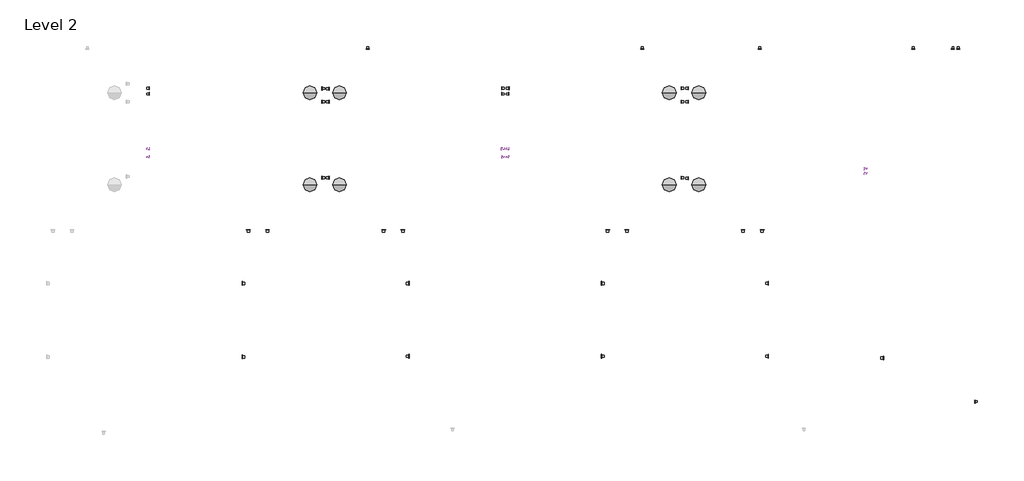
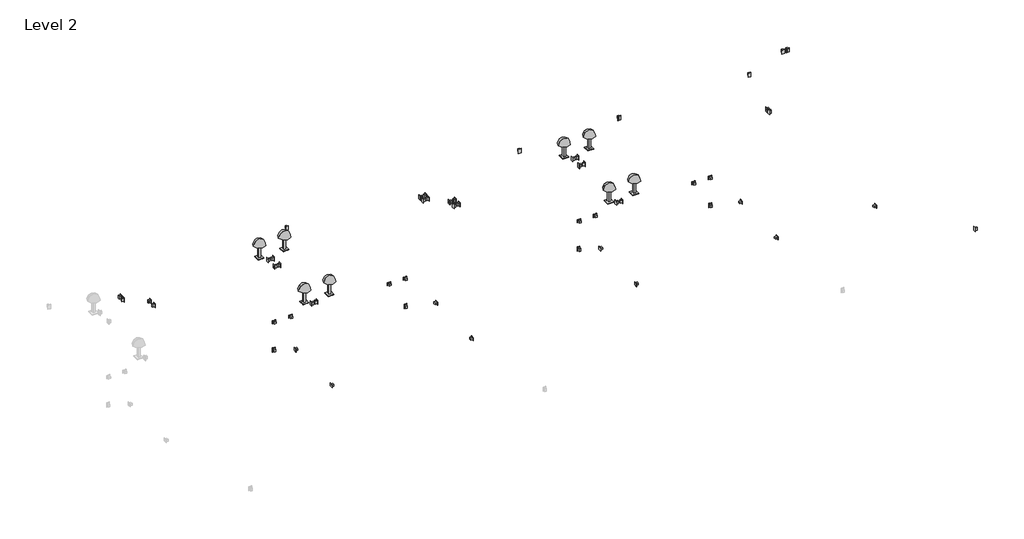
# One storey, part 2 of 2: 37 proxies, 17 switching devices, 8 light fixtures.
# Revit data of these elements (continued)
# Type "Table Lamp - Hemispheric : 60W - 230V" (continued)
#   built-in parameter 1150112 = 1 (stored number, unit not read)
#   built-in parameter 1150114 = 1 (stored number, unit not read)
#   built-in parameter 1150107 = 2800 (stored number, unit not read)
#   built-in parameter 1150106 = 0.680387 (stored number, unit not read)
#   built-in parameter 1150104 = 1.32387 (stored number, unit not read)
#   Ballast Voltage = 230 V
#   built-in parameter 1114218 = 1 (stored number, unit not read)
#   built-in parameter 1150133 = 10 (stored number, unit not read)
#   Lumens = 855 lm
#   Apparent Load = 60 VA
#   COBie.Type = yes
#   built-in parameter 1150134 = 4
#   built-in parameter 1150137 = 1
#   Color Filter = 16777215
#   Ballast Number of Poles = 1
#   T.L. Material = Wood - Birch
#   Mount Material = Metal - Chrome
#   Load Classification = Lighting - Dwelling Unit
#   Shade Material = Glass - Frosted
#   Base Material = Wood - Birch
#   Dimming Lamp Color Temperature Shift = (empty or 0)
#   Default Elevation = 0
#   Wattage Comments = ""
# Type "Lighting Switches One Way : One Way Switch"
#   Type Mark = "Lighting Switches One Way"
#   Classification.OmniClass.21.Number = "21-04 50 40 10"
#   Classification.OmniClass.21.Description = "Lighting Control"
#   Classification.UniFormat.II.Description = "Lighting Control"
#   Classification.OmniClass.23.Number = "23-35 37 00"
#   Classification.OmniClass.23.Description = "Electrical Switches"
#   Classification.UniFormat.II.Number = "D5040.10"
#   COBie.Type.CreatedBy = "info@mma.ie"
#   COBie.Type.CreatedOn = "2017-07-25T10:15:16"
#   COBie.Type.Name = "Lighting Switches One Way"
#   COBie.Type.Category = "23-35 37 00 : Electrical Switches"
#   COBie.Type.Description = "Lighting Switches One Way_One Way Switch"
#   COBie.Type.AssetType = "Fixed"
#   COBie.Type.Manufacturer = ""
#   COBie.Type.ModelNumber = ""
#   Label = ""
#   Keynote = "26 36 13.A"
#   COBie.Type.ReplacementCost = 0
#   Switch Voltage [instance default] = 230 V
#   Default Elevation = 1200 mm
#   Apparent Load = 0 VA
#   1.W.S. Width = 86 mm
#   1.W.S. Height = 86 mm
#   1.W.S. Depth = 59 mm
#   COBie.Type = yes
#   Visibility 7 = no
#   Visibility 6 = no
#   Visibility 5 = yes
#   Visibility 4 = no
#   Visibility 3 = no
#   Visibility 2 = no
#   Visibility 1 = no
#   Ballast Number of Poles = 1
#   Load Classification = Other
#   1.W.S. Material = Metal - Chrome
# Type "Lighting Switches Two Way : Two Way Switch"
#   Type Mark = "Lighting Switches Two Way"
#   Classification.OmniClass.23.Number = "23-35 37 00"
#   Classification.OmniClass.23.Description = "Electrical Switches"
#   COBie.Type.CreatedBy = "info@mma.ie"
#   COBie.Type.CreatedOn = "2017-07-25T10:15:16"
#   COBie.Type.Name = "Lighting Switches Two Way"
#   COBie.Type.Category = "23-35 37 00 : Electrical Switches"
#   COBie.Type.Description = "Lighting Switches Two Way_Two Way Switch"
#   COBie.Type.AssetType = "Fixed"
#   COBie.Type.Manufacturer = ""
#   COBie.Type.ModelNumber = ""
#   Label = ""
#   Keynote = "26 36 13.B"
#   COBie.Type.ReplacementCost = 0
#   Switch Voltage [instance default] = 230 V
#   Default Elevation = 1200 mm
#   Apparent Load = 0 VA
#   2.W.S. Width = 86 mm
#   2.W.S. Height = 86 mm
#   2.W.S. Depth = 59 mm
#   COBie.Type = yes
#   Visibility 7 = no
#   Visibility 6 = no
#   Visibility 5 = yes
#   Visibility 4 = no
#   Visibility 3 = no
#   Visibility 2 = no
#   Visibility 1 = no
#   Ballast Number of Poles = 1
#   Load Classification = Other
#   2.W.S. Material = Metal - Chrome
# Element 1 (IfcBuildingElementProxy, "M_Duplex Receptacle - Top Switched : Standard")
#   Mark = "1"
#   COBie.CreatedBy = "info@mma.ie"
#   COBie.CreatedOn = "2017-07-25T10:15:16"
#   COBie.Component.Name = "M_Duplex Receptacle - Top Switched_1"
#   COBie.Component.Space = "213"
#   COBie.Component.Description = "M_Duplex Receptacle - Top Switched: Standard"
#   Notes = "n/a"
#   COBie = yes
#   Phase Created = New Construction
# Element 2 (IfcBuildingElementProxy, "M_Duplex Receptacle - Top Switched : Standard")
#   Mark = "2"
#   COBie.CreatedBy = "info@mma.ie"
#   COBie.CreatedOn = "2017-07-25T10:15:16"
#   COBie.Component.Name = "M_Duplex Receptacle - Top Switched_2"
#   COBie.Component.Space = "215"
#   COBie.Component.Description = "M_Duplex Receptacle - Top Switched: Standard"
#   Notes = "n/a"
#   COBie = yes
#   Phase Created = New Construction
# Element 3 (IfcBuildingElementProxy, "M_Duplex Receptacle - Top Switched : Standard")
#   Mark = "3"
#   COBie.CreatedBy = "info@mma.ie"
#   COBie.CreatedOn = "2017-07-25T10:15:16"
#   COBie.Component.Name = "M_Duplex Receptacle - Top Switched_3"
#   COBie.Component.Space = "215"
#   COBie.Component.Description = "M_Duplex Receptacle - Top Switched: Standard"
#   Notes = "n/a"
#   COBie = yes
#   Phase Created = New Construction
# Element 4 (IfcBuildingElementProxy, "M_Duplex Receptacle - Top Switched : Standard")
#   Mark = "4"
#   COBie.CreatedBy = "info@mma.ie"
#   COBie.CreatedOn = "2017-07-25T10:15:16"
#   COBie.Component.Name = "M_Duplex Receptacle - Top Switched_4"
#   COBie.Component.Space = "211"
#   COBie.Component.Description = "M_Duplex Receptacle - Top Switched: Standard"
#   Notes = "n/a"
#   COBie = yes
#   Phase Created = New Construction
# Element 5 (IfcBuildingElementProxy, "M_Duplex Receptacle - Top Switched : Standard")
#   Mark = "5"
#   COBie.CreatedBy = "info@mma.ie"
#   COBie.CreatedOn = "2017-07-25T10:15:16"
#   COBie.Component.Name = "M_Duplex Receptacle - Top Switched_5"
#   COBie.Component.Space = "211"
#   COBie.Component.Description = "M_Duplex Receptacle - Top Switched: Standard"
#   Notes = "n/a"
#   COBie = yes
#   Phase Created = New Construction
# Element 6 (IfcBuildingElementProxy, "M_Duplex Receptacle - Top Switched : Standard")
#   Mark = "6"
#   COBie.CreatedBy = "info@mma.ie"
#   COBie.CreatedOn = "2017-07-25T10:15:16"
#   COBie.Component.Name = "M_Duplex Receptacle - Top Switched_6"
#   COBie.Component.Space = "209"
#   COBie.Component.Description = "M_Duplex Receptacle - Top Switched: Standard"
#   Notes = "n/a"
#   COBie = yes
#   Phase Created = New Construction
# Element 7 (IfcBuildingElementProxy, "M_Duplex Receptacle - Top Switched : Standard")
#   Mark = "11"
#   COBie.CreatedBy = "info@mma.ie"
#   COBie.CreatedOn = "2017-07-25T10:15:16"
#   COBie.Component.Name = "M_Duplex Receptacle - Top Switched_11"
#   COBie.Component.Space = "209"
#   COBie.Component.Description = "M_Duplex Receptacle - Top Switched: Standard"
#   Notes = "n/a"
#   COBie = yes
#   Phase Created = New Construction
# Element 8 (IfcBuildingElementProxy, "M_Duplex Receptacle - Top Switched : Standard")
#   Mark = "12"
#   COBie.CreatedBy = "info@mma.ie"
#   COBie.CreatedOn = "2017-07-25T10:15:16"
#   COBie.Component.Name = "M_Duplex Receptacle - Top Switched_12"
#   COBie.Component.Space = "213"
#   COBie.Component.Description = "M_Duplex Receptacle - Top Switched: Standard"
#   Notes = "n/a"
#   COBie = yes
#   Phase Created = New Construction
# Element 9 (IfcBuildingElementProxy, "M_Duplex Receptacle - Top Switched : Standard")
#   Mark = "13"
#   COBie.CreatedBy = "info@mma.ie"
#   COBie.CreatedOn = "2017-07-25T10:15:16"
#   COBie.Component.Name = "M_Duplex Receptacle - Top Switched_13"
#   COBie.Component.Space = "213"
#   COBie.Component.Description = "M_Duplex Receptacle - Top Switched: Standard"
#   Notes = "n/a"
#   COBie = yes
#   Phase Created = New Construction
# Element 10 (IfcBuildingElementProxy, "M_Duplex Receptacle - Top Switched : Standard")
#   Mark = "14"
#   COBie.CreatedBy = "info@mma.ie"
#   COBie.CreatedOn = "2017-07-25T10:15:16"
#   COBie.Component.Name = "M_Duplex Receptacle - Top Switched_14"
#   COBie.Component.Space = "215"
#   COBie.Component.Description = "M_Duplex Receptacle - Top Switched: Standard"
#   Notes = "n/a"
#   COBie = yes
#   Phase Created = New Construction
# Element 11 (IfcBuildingElementProxy, "M_Receptacle - 220V : Standard")
#   Mark = "1"
#   COBie.CreatedBy = "info@mma.ie"
#   COBie.CreatedOn = "2017-07-25T10:15:16"
#   COBie.Component.Name = "M_Receptacle - 220V_1"
#   COBie.Component.Space = "215"
#   COBie.Component.Description = "M_Receptacle - 220V: Standard"
#   Notes = "n/a"
#   COBie = yes
#   Phase Created = New Construction
# Element 12 (IfcBuildingElementProxy, "M_Receptacle - 220V : Standard")
#   Mark = "2"
#   COBie.CreatedBy = "info@mma.ie"
#   COBie.CreatedOn = "2017-07-25T10:15:16"
#   COBie.Component.Name = "M_Receptacle - 220V_2"
#   COBie.Component.Space = "215"
#   COBie.Component.Description = "M_Receptacle - 220V: Standard"
#   Notes = "n/a"
#   COBie = yes
#   Phase Created = New Construction
# Element 13 (IfcBuildingElementProxy, "M_Receptacle - 220V : Standard")
#   Mark = "3"
#   COBie.CreatedBy = "info@mma.ie"
#   COBie.CreatedOn = "2017-07-25T10:15:16"
#   COBie.Component.Name = "M_Receptacle - 220V_3"
#   COBie.Component.Space = "215"
#   COBie.Component.Description = "M_Receptacle - 220V: Standard"
#   Notes = "n/a"
#   COBie = yes
#   Phase Created = New Construction
# Element 14 (IfcBuildingElementProxy, "M_Receptacle - 220V : Standard")
#   Mark = "4"
#   COBie.CreatedBy = "info@mma.ie"
#   COBie.CreatedOn = "2017-07-25T10:15:16"
#   COBie.Component.Name = "M_Receptacle - 220V_4"
#   COBie.Component.Space = "215"
#   COBie.Component.Description = "M_Receptacle - 220V: Standard"
#   Notes = "n/a"
#   COBie = yes
#   Phase Created = New Construction
# Element 15 (IfcBuildingElementProxy, "M_Receptacle - 220V : Standard")
#   Mark = "5"
#   COBie.CreatedBy = "info@mma.ie"
#   COBie.CreatedOn = "2017-07-25T10:15:16"
#   COBie.Component.Name = "M_Receptacle - 220V_5"
#   COBie.Component.Space = "213"
#   COBie.Component.Description = "M_Receptacle - 220V: Standard"
#   Notes = "n/a"
#   COBie = yes
#   Phase Created = New Construction
# Element 16 (IfcBuildingElementProxy, "M_Receptacle - 220V : Standard")
#   Mark = "6"
#   COBie.CreatedBy = "info@mma.ie"
#   COBie.CreatedOn = "2017-07-25T10:15:16"
#   COBie.Component.Name = "M_Receptacle - 220V_6"
#   COBie.Component.Space = "213"
#   COBie.Component.Description = "M_Receptacle - 220V: Standard"
#   Notes = "n/a"
#   COBie = yes
#   Phase Created = New Construction
# Element 17 (IfcBuildingElementProxy, "M_Receptacle - 220V : Standard")
#   Mark = "7"
#   COBie.CreatedBy = "info@mma.ie"
#   COBie.CreatedOn = "2017-07-25T10:15:16"
#   COBie.Component.Name = "M_Receptacle - 220V_7"
#   COBie.Component.Space = "213"
#   COBie.Component.Description = "M_Receptacle - 220V: Standard"
#   Notes = "n/a"
#   COBie = yes
#   Phase Created = New Construction
# Element 18 (IfcBuildingElementProxy, "M_Receptacle - 220V : Standard")
#   Mark = "8"
#   COBie.CreatedBy = "info@mma.ie"
#   COBie.CreatedOn = "2017-07-25T10:15:16"
#   COBie.Component.Name = "M_Receptacle - 220V_8"
#   COBie.Component.Space = "211"
#   COBie.Component.Description = "M_Receptacle - 220V: Standard"
#   Notes = "n/a"
#   COBie = yes
#   Phase Created = New Construction
# Element 19 (IfcBuildingElementProxy, "M_Receptacle - 220V : Standard")
#   Mark = "9"
#   COBie.CreatedBy = "info@mma.ie"
#   COBie.CreatedOn = "2017-07-25T10:15:16"
#   COBie.Component.Name = "M_Receptacle - 220V_9"
#   COBie.Component.Space = "211"
#   COBie.Component.Description = "M_Receptacle - 220V: Standard"
#   Notes = "n/a"
#   COBie = yes
#   Phase Created = New Construction
# Element 20 (IfcBuildingElementProxy, "M_Receptacle - 220V : Standard")
#   Mark = "10"
#   COBie.CreatedBy = "info@mma.ie"
#   COBie.CreatedOn = "2017-07-25T10:15:16"
#   COBie.Component.Name = "M_Receptacle - 220V_10"
#   COBie.Component.Space = "211"
#   COBie.Component.Description = "M_Receptacle - 220V: Standard"
#   Notes = "n/a"
#   COBie = yes
#   Phase Created = New Construction
# Element 21 (IfcBuildingElementProxy, "M_Receptacle - 220V : Standard")
#   Mark = "11"
#   COBie.CreatedBy = "info@mma.ie"
#   COBie.CreatedOn = "2017-07-25T10:15:16"
#   COBie.Component.Name = "M_Receptacle - 220V_11"
#   COBie.Component.Space = "211"
#   COBie.Component.Description = "M_Receptacle - 220V: Standard"
#   Notes = "n/a"
#   COBie = yes
#   Phase Created = New Construction
# Element 22 (IfcBuildingElementProxy, "M_Receptacle - 220V : Standard")
#   Mark = "12"
#   COBie.CreatedBy = "info@mma.ie"
#   COBie.CreatedOn = "2017-07-25T10:15:16"
#   COBie.Component.Name = "M_Receptacle - 220V_12"
#   COBie.Component.Space = "209"
#   COBie.Component.Description = "M_Receptacle - 220V: Standard"
#   Notes = "n/a"
#   COBie = yes
#   Phase Created = New Construction
# Element 23 (IfcBuildingElementProxy, "M_Receptacle - 220V : Standard")
#   Mark = "13"
#   COBie.CreatedBy = "info@mma.ie"
#   COBie.CreatedOn = "2017-07-25T10:15:16"
#   COBie.Component.Name = "M_Receptacle - 220V_13"
#   COBie.Component.Space = "209"
#   COBie.Component.Description = "M_Receptacle - 220V: Standard"
#   Notes = "n/a"
#   COBie = yes
#   Phase Created = New Construction
# Element 24 (IfcBuildingElementProxy, "M_Receptacle - 220V : Standard")
#   Mark = "14"
#   COBie.CreatedBy = "info@mma.ie"
#   COBie.CreatedOn = "2017-07-25T10:15:16"
#   COBie.Component.Name = "M_Receptacle - 220V_14"
#   COBie.Component.Space = "209"
#   COBie.Component.Description = "M_Receptacle - 220V: Standard"
#   Notes = "n/a"
#   COBie = yes
#   Phase Created = New Construction
# Element 25 (IfcBuildingElementProxy, "M_Receptacle - 220V : Standard")
#   Mark = "37"
#   COBie.CreatedBy = "info@mma.ie"
#   COBie.CreatedOn = "2017-07-25T10:15:16"
#   COBie.Component.Name = "M_Receptacle - 220V_37"
#   COBie.Component.Space = "219"
#   COBie.Component.Description = "M_Receptacle - 220V: Standard"
#   Notes = "n/a"
#   COBie = yes
#   Phase Created = New Construction
# Element 26 (IfcBuildingElementProxy, "M_Receptacle - DATA socket : Standard")
#   Mark = "6"
#   COBie.CreatedBy = "info@mma.ie"
#   COBie.CreatedOn = "2017-07-25T10:15:16"
#   COBie.Component.Name = "M_Receptacle - DATA socket_6"
#   COBie.Component.Space = "209"
#   COBie.Component.Description = "M_Receptacle - DATA socket: Standard"
#   Notes = "n/a"
#   COBie = yes
#   Phase Created = New Construction
# Element 27 (IfcBuildingElementProxy, "M_Receptacle - DATA socket : Standard")
#   Mark = "7"
#   COBie.CreatedBy = "info@mma.ie"
#   COBie.CreatedOn = "2017-07-25T10:15:16"
#   COBie.Component.Name = "M_Receptacle - DATA socket_7"
#   COBie.Component.Space = "209"
#   COBie.Component.Description = "M_Receptacle - DATA socket: Standard"
#   Notes = "n/a"
#   COBie = yes
#   Phase Created = New Construction
# Element 28 (IfcBuildingElementProxy, "M_Receptacle - DATA socket : Standard")
#   Mark = "8"
#   COBie.CreatedBy = "info@mma.ie"
#   COBie.CreatedOn = "2017-07-25T10:15:16"
#   COBie.Component.Name = "M_Receptacle - DATA socket_8"
#   COBie.Component.Space = "211"
#   COBie.Component.Description = "M_Receptacle - DATA socket: Standard"
#   Notes = "n/a"
#   COBie = yes
#   Phase Created = New Construction
# Element 29 (IfcBuildingElementProxy, "M_Receptacle - DATA socket : Standard")
#   Mark = "9"
#   COBie.CreatedBy = "info@mma.ie"
#   COBie.CreatedOn = "2017-07-25T10:15:16"
#   COBie.Component.Name = "M_Receptacle - DATA socket_9"
#   COBie.Component.Space = "211"
#   COBie.Component.Description = "M_Receptacle - DATA socket: Standard"
#   Notes = "n/a"
#   COBie = yes
#   Phase Created = New Construction
# Element 30 (IfcBuildingElementProxy, "M_Receptacle - DATA socket : Standard")
#   Mark = "10"
#   COBie.CreatedBy = "info@mma.ie"
#   COBie.CreatedOn = "2017-07-25T10:15:16"
#   COBie.Component.Name = "M_Receptacle - DATA socket_10"
#   COBie.Component.Space = "213"
#   COBie.Component.Description = "M_Receptacle - DATA socket: Standard"
#   Notes = "n/a"
#   COBie = yes
#   Phase Created = New Construction
# Element 31 (IfcBuildingElementProxy, "M_Receptacle - DATA socket : Standard")
#   Mark = "11"
#   COBie.CreatedBy = "info@mma.ie"
#   COBie.CreatedOn = "2017-07-25T10:15:16"
#   COBie.Component.Name = "M_Receptacle - DATA socket_11"
#   COBie.Component.Space = "215"
#   COBie.Component.Description = "M_Receptacle - DATA socket: Standard"
#   Notes = "n/a"
#   COBie = yes
#   Phase Created = New Construction
# Element 32 (IfcBuildingElementProxy, "M_Receptacle - DATA socket : Standard")
#   Mark = "18"
#   COBie.CreatedBy = "info@mma.ie"
#   COBie.CreatedOn = "2017-07-25T10:15:16"
#   COBie.Component.Name = "M_Receptacle - DATA socket_18"
#   COBie.Component.Space = "213"
#   COBie.Component.Description = "M_Receptacle - DATA socket: Standard"
#   Notes = "n/a"
#   COBie = yes
#   Phase Created = New Construction
# Element 33 (IfcBuildingElementProxy, "M_Receptacle - DATA socket : Standard")
#   Mark = "21"
#   COBie.CreatedBy = "info@mma.ie"
#   COBie.CreatedOn = "2017-07-25T10:15:16"
#   COBie.Component.Name = "M_Receptacle - DATA socket_21"
#   COBie.Component.Space = "215"
#   COBie.Component.Description = "M_Receptacle - DATA socket: Standard"
#   Notes = "n/a"
#   COBie = yes
#   Phase Created = New Construction
# Element 34 (IfcBuildingElementProxy, "M_Receptacle -TV /Satellite Socket : Standard")
#   Mark = "3"
#   COBie.CreatedBy = "info@mma.ie"
#   COBie.CreatedOn = "2017-07-25T10:15:16"
#   COBie.Component.Name = "M_Receptacle -TV_3"
#   COBie.Component.Space = "211"
#   COBie.Component.Description = "M_Receptacle -TV: Standard"
#   Notes = "n/a"
#   COBie = yes
#   Phase Created = New Construction
# Element 35 (IfcBuildingElementProxy, "M_Receptacle -TV /Satellite Socket : Standard")
#   Mark = "4"
#   COBie.CreatedBy = "info@mma.ie"
#   COBie.CreatedOn = "2017-07-25T10:15:16"
#   COBie.Component.Name = "M_Receptacle -TV_4"
#   COBie.Component.Space = "213"
#   COBie.Component.Description = "M_Receptacle -TV: Standard"
#   Notes = "n/a"
#   COBie = yes
#   Phase Created = New Construction
# Element 36 (IfcBuildingElementProxy, "M_Receptacle -TV /Satellite Socket : Standard")
#   Mark = "5"
#   COBie.CreatedBy = "info@mma.ie"
#   COBie.CreatedOn = "2017-07-25T10:15:16"
#   COBie.Component.Name = "M_Receptacle -TV_5"
#   COBie.Component.Space = "215"
#   COBie.Component.Description = "M_Receptacle -TV: Standard"
#   Notes = "n/a"
#   COBie = yes
#   Phase Created = New Construction
# Element 37 (IfcBuildingElementProxy, "M_Receptacle -TV /Satellite Socket : Standard")
#   Mark = "6"
#   COBie.CreatedBy = "info@mma.ie"
#   COBie.CreatedOn = "2017-07-25T10:15:16"
#   COBie.Component.Name = "M_Receptacle -TV_6"
#   COBie.Component.Space = "209"
#   COBie.Component.Description = "M_Receptacle -TV: Standard"
#   Notes = "n/a"
#   COBie = yes
#   Phase Created = New Construction
# Element 38 (IfcLightFixture, "Table Lamp - Hemispheric : 60W - 230V")
#   Comments = "Lamps"
#   Mark = "1"
#   COBie.CreatedBy = "info@mma.ie"
#   COBie.CreatedOn = "2017-07-25T10:15:16"
#   COBie.Component.Name = "Table Lamp - Hemispheric_1"
#   COBie.Component.Space = "211"
#   COBie.Component.Description = "Table Lamp - Hemispheric: 60W - 230V"
#   Notes = "n/a"
#   Floor Level = "Level 2"
#   COBie = yes
#   Phase Created = New Construction
#   Materials on its faces: "Metal - Chrome", "Glass - Frosted", "Wood - Birch"
# Element 39 (IfcLightFixture, "Table Lamp - Hemispheric : 60W - 230V")
#   Comments = "Lamps"
#   Mark = "2"
#   COBie.CreatedBy = "info@mma.ie"
#   COBie.CreatedOn = "2017-07-25T10:15:16"
#   COBie.Component.Name = "Table Lamp - Hemispheric_2"
#   COBie.Component.Space = "211"
#   COBie.Component.Description = "Table Lamp - Hemispheric: 60W - 230V"
#   Notes = "n/a"
#   Floor Level = "Level 2"
#   COBie = yes
#   Phase Created = New Construction
#   Materials on its faces: "Metal - Chrome", "Glass - Frosted", "Wood - Birch"
# Element 40 (IfcLightFixture, "Table Lamp - Hemispheric : 60W - 230V")
#   Comments = "Lamps"
#   Mark = "3"
#   COBie.CreatedBy = "info@mma.ie"
#   COBie.CreatedOn = "2017-07-25T10:15:16"
#   COBie.Component.Name = "Table Lamp - Hemispheric_3"
#   COBie.Component.Space = "209"
#   COBie.Component.Description = "Table Lamp - Hemispheric: 60W - 230V"
#   Notes = "n/a"
#   Floor Level = "Level 2"
#   COBie = yes
#   Phase Created = New Construction
#   Materials on its faces: "Metal - Chrome", "Glass - Frosted", "Wood - Birch"
# Element 41 (IfcLightFixture, "Table Lamp - Hemispheric : 60W - 230V")
#   Comments = "Lamps"
#   Mark = "4"
#   COBie.CreatedBy = "info@mma.ie"
#   COBie.CreatedOn = "2017-07-25T10:15:16"
#   COBie.Component.Name = "Table Lamp - Hemispheric_4"
#   COBie.Component.Space = "209"
#   COBie.Component.Description = "Table Lamp - Hemispheric: 60W - 230V"
#   Notes = "n/a"
#   Floor Level = "Level 2"
#   COBie = yes
#   Phase Created = New Construction
#   Materials on its faces: "Metal - Chrome", "Glass - Frosted", "Wood - Birch"
# Element 42 (IfcLightFixture, "Table Lamp - Hemispheric : 60W - 230V")
#   Comments = "Lamps"
#   Mark = "11"
#   COBie.CreatedBy = "info@mma.ie"
#   COBie.CreatedOn = "2017-07-25T10:15:16"
#   COBie.Component.Name = "Table Lamp - Hemispheric_11"
#   COBie.Component.Space = "213"
#   COBie.Component.Description = "Table Lamp - Hemispheric: 60W - 230V"
#   Notes = "n/a"
#   Floor Level = "Level 2"
#   COBie = yes
#   Phase Created = New Construction
#   Materials on its faces: "Metal - Chrome", "Glass - Frosted", "Wood - Birch"
# Element 43 (IfcLightFixture, "Table Lamp - Hemispheric : 60W - 230V")
#   Comments = "Lamps"
#   Mark = "12"
#   COBie.CreatedBy = "info@mma.ie"
#   COBie.CreatedOn = "2017-07-25T10:15:16"
#   COBie.Component.Name = "Table Lamp - Hemispheric_12"
#   COBie.Component.Space = "213"
#   COBie.Component.Description = "Table Lamp - Hemispheric: 60W - 230V"
#   Notes = "n/a"
#   Floor Level = "Level 2"
#   COBie = yes
#   Phase Created = New Construction
#   Materials on its faces: "Metal - Chrome", "Glass - Frosted", "Wood - Birch"
# Element 44 (IfcLightFixture, "Table Lamp - Hemispheric : 60W - 230V")
#   Comments = "Lamps"
#   Mark = "13"
#   COBie.CreatedBy = "info@mma.ie"
#   COBie.CreatedOn = "2017-07-25T10:15:16"
#   COBie.Component.Name = "Table Lamp - Hemispheric_13"
#   COBie.Component.Space = "215"
#   COBie.Component.Description = "Table Lamp - Hemispheric: 60W - 230V"
#   Notes = "n/a"
#   Floor Level = "Level 2"
#   COBie = yes
#   Phase Created = New Construction
#   Materials on its faces: "Metal - Chrome", "Glass - Frosted", "Wood - Birch"
# Element 45 (IfcLightFixture, "Table Lamp - Hemispheric : 60W - 230V")
#   Comments = "Lamps"
#   Mark = "14"
#   COBie.CreatedBy = "info@mma.ie"
#   COBie.CreatedOn = "2017-07-25T10:15:16"
#   COBie.Component.Name = "Table Lamp - Hemispheric_14"
#   COBie.Component.Space = "215"
#   COBie.Component.Description = "Table Lamp - Hemispheric: 60W - 230V"
#   Notes = "n/a"
#   Floor Level = "Level 2"
#   COBie = yes
#   Phase Created = New Construction
#   Materials on its faces: "Metal - Chrome", "Glass - Frosted", "Wood - Birch"
# Element 46 (IfcSwitchingDevice, "Lighting Switches One Way : One Way Switch")
#   Comments = "Switch"
#   Mark = "10"
#   COBie.CreatedBy = "info@mma.ie"
#   COBie.CreatedOn = "2017-07-25T10:15:16"
#   COBie.Component.Name = "Lighting Switches One Way_10"
#   COBie.Component.Space = "213"
#   COBie.Component.Description = "Lighting Switches One Way: One Way Switch"
#   Notes = "n/a"
#   Floor Level = "Level 2"
#   COBie = yes
#   Phase Created = New Construction
# Element 47 (IfcSwitchingDevice, "Lighting Switches One Way : One Way Switch")
#   Comments = "Switch"
#   Mark = "11"
#   COBie.CreatedBy = "info@mma.ie"
#   COBie.CreatedOn = "2017-07-25T10:15:16"
#   COBie.Component.Name = "Lighting Switches One Way_11"
#   COBie.Component.Space = "215"
#   COBie.Component.Description = "Lighting Switches One Way: One Way Switch"
#   Notes = "n/a"
#   Floor Level = "Level 2"
#   COBie = yes
#   Phase Created = New Construction
# Element 48 (IfcSwitchingDevice, "Lighting Switches One Way : One Way Switch")
#   Comments = "Switch"
#   Mark = "12"
#   COBie.CreatedBy = "info@mma.ie"
#   COBie.CreatedOn = "2017-07-25T10:15:16"
#   COBie.Component.Name = "Lighting Switches One Way_12"
#   COBie.Component.Space = "211"
#   COBie.Component.Description = "Lighting Switches One Way: One Way Switch"
#   Notes = "n/a"
#   Floor Level = "Level 2"
#   COBie = yes
#   Phase Created = New Construction
# Element 49 (IfcSwitchingDevice, "Lighting Switches One Way : One Way Switch")
#   Comments = "Switch"
#   Mark = "13"
#   COBie.CreatedBy = "info@mma.ie"
#   COBie.CreatedOn = "2017-07-25T10:15:16"
#   COBie.Component.Name = "Lighting Switches One Way_13"
#   COBie.Component.Space = "209"
#   COBie.Component.Description = "Lighting Switches One Way: One Way Switch"
#   Notes = "n/a"
#   Floor Level = "Level 2"
#   COBie = yes
#   Phase Created = New Construction
# Element 50 (IfcSwitchingDevice, "Lighting Switches One Way : One Way Switch")
#   Comments = "Switch"
#   Mark = "16"
#   COBie.CreatedBy = "info@mma.ie"
#   COBie.CreatedOn = "2017-07-25T10:15:16"
#   COBie.Component.Name = "Lighting Switches One Way_16"
#   COBie.Component.Space = "209"
#   COBie.Component.Description = "Lighting Switches One Way: One Way Switch"
#   Notes = "n/a"
#   Floor Level = "Level 2"
#   COBie = yes
#   Phase Created = New Construction
# Element 51 (IfcSwitchingDevice, "Lighting Switches One Way : One Way Switch")
#   Comments = "Switch"
#   Mark = "17"
#   COBie.CreatedBy = "info@mma.ie"
#   COBie.CreatedOn = "2017-07-25T10:15:16"
#   COBie.Component.Name = "Lighting Switches One Way_17"
#   COBie.Component.Space = "209"
#   COBie.Component.Description = "Lighting Switches One Way: One Way Switch"
#   Notes = "n/a"
#   Floor Level = "Level 2"
#   COBie = yes
#   Phase Created = New Construction
# Element 52 (IfcSwitchingDevice, "Lighting Switches One Way : One Way Switch")
#   Comments = "Switch"
#   Mark = "18"
#   COBie.CreatedBy = "info@mma.ie"
#   COBie.CreatedOn = "2017-07-25T10:15:16"
#   COBie.Component.Name = "Lighting Switches One Way_18"
#   COBie.Component.Space = "213"
#   COBie.Component.Description = "Lighting Switches One Way: One Way Switch"
#   Notes = "n/a"
#   Floor Level = "Level 2"
#   COBie = yes
#   Phase Created = New Construction
# Element 53 (IfcSwitchingDevice, "Lighting Switches One Way : One Way Switch")
#   Comments = "Switch"
#   Mark = "19"
#   COBie.CreatedBy = "info@mma.ie"
#   COBie.CreatedOn = "2017-07-25T10:15:16"
#   COBie.Component.Name = "Lighting Switches One Way_19"
#   COBie.Component.Space = "215"
#   COBie.Component.Description = "Lighting Switches One Way: One Way Switch"
#   Notes = "n/a"
#   Floor Level = "Level 2"
#   COBie = yes
#   Phase Created = New Construction
# Element 54 (IfcSwitchingDevice, "Lighting Switches One Way : One Way Switch")
#   Comments = "Switch"
#   Mark = "20"
#   COBie.CreatedBy = "info@mma.ie"
#   COBie.CreatedOn = "2017-07-25T10:15:16"
#   COBie.Component.Name = "Lighting Switches One Way_20"
#   COBie.Component.Space = "215"
#   COBie.Component.Description = "Lighting Switches One Way: One Way Switch"
#   Notes = "n/a"
#   Floor Level = "Level 2"
#   COBie = yes
#   Phase Created = New Construction
# Element 55 (IfcSwitchingDevice, "Lighting Switches One Way : One Way Switch")
#   Comments = "Switch"
#   Mark = "28"
#   COBie.CreatedBy = "info@mma.ie"
#   COBie.CreatedOn = "2017-07-25T10:15:16"
#   COBie.Component.Name = "Lighting Switches One Way_28"
#   COBie.Component.Space = "209"
#   COBie.Component.Description = "Lighting Switches One Way: One Way Switch"
#   Notes = "n/a"
#   Floor Level = "Level 2"
#   COBie = yes
#   Phase Created = New Construction
# Element 56 (IfcSwitchingDevice, "Lighting Switches One Way : One Way Switch")
#   Comments = "Switch"
#   Mark = "29"
#   COBie.CreatedBy = "info@mma.ie"
#   COBie.CreatedOn = "2017-07-25T10:15:16"
#   COBie.Component.Name = "Lighting Switches One Way_29"
#   COBie.Component.Space = "211"
#   COBie.Component.Description = "Lighting Switches One Way: One Way Switch"
#   Notes = "n/a"
#   Floor Level = "Level 2"
#   COBie = yes
#   Phase Created = New Construction
# Element 57 (IfcSwitchingDevice, "Lighting Switches One Way : One Way Switch")
#   Comments = "Switch"
#   Mark = "30"
#   COBie.CreatedBy = "info@mma.ie"
#   COBie.CreatedOn = "2017-07-25T10:15:16"
#   COBie.Component.Name = "Lighting Switches One Way_30"
#   COBie.Component.Space = "213"
#   COBie.Component.Description = "Lighting Switches One Way: One Way Switch"
#   Notes = "n/a"
#   Floor Level = "Level 2"
#   COBie = yes
#   Phase Created = New Construction
# Element 58 (IfcSwitchingDevice, "Lighting Switches One Way : One Way Switch")
#   Comments = "Switch"
#   Mark = "31"
#   COBie.CreatedBy = "info@mma.ie"
#   COBie.CreatedOn = "2017-07-25T10:15:16"
#   COBie.Component.Name = "Lighting Switches One Way_31"
#   COBie.Component.Space = "215"
#   COBie.Component.Description = "Lighting Switches One Way: One Way Switch"
#   Notes = "n/a"
#   Floor Level = "Level 2"
#   COBie = yes
#   Phase Created = New Construction
# Element 59 (IfcSwitchingDevice, "Lighting Switches One Way : One Way Switch")
#   Comments = "Switch"
#   Mark = "49"
#   COBie.CreatedBy = "info@mma.ie"
#   COBie.CreatedOn = "2017-07-25T10:15:16"
#   COBie.Component.Name = "Lighting Switches One Way_49"
#   COBie.Component.Space = "211"
#   COBie.Component.Description = "Lighting Switches One Way: One Way Switch"
#   Notes = "n/a"
#   Floor Level = "Level 2"
#   COBie = yes
#   Phase Created = New Construction
# Element 60 (IfcSwitchingDevice, "Lighting Switches One Way : One Way Switch")
#   Comments = "Switch"
#   Mark = "50"
#   COBie.CreatedBy = "info@mma.ie"
#   COBie.CreatedOn = "2017-07-25T10:15:16"
#   COBie.Component.Name = "Lighting Switches One Way_50"
#   COBie.Component.Space = "211"
#   COBie.Component.Description = "Lighting Switches One Way: One Way Switch"
#   Notes = "n/a"
#   Floor Level = "Level 2"
#   COBie = yes
#   Phase Created = New Construction
# Element 61 (IfcSwitchingDevice, "Lighting Switches One Way : One Way Switch")
#   Comments = "Switch"
#   Mark = "6"
#   COBie.CreatedBy = "info@mma.ie"
#   COBie.CreatedOn = "2017-07-25T10:15:16"
#   COBie.Component.Name = "Lighting Switches One Way_6"
#   COBie.Component.Space = "213"
#   COBie.Component.Description = "Lighting Switches One Way: One Way Switch"
#   Notes = "n/a"
#   Floor Level = "Level 2"
#   COBie = yes
#   Phase Created = New Construction
# Element 62 (IfcSwitchingDevice, "Lighting Switches Two Way : Two Way Switch")
#   Mark = "7"
#   COBie.CreatedBy = "info@mma.ie"
#   COBie.CreatedOn = "2017-07-25T10:15:16"
#   COBie.Component.Name = "Lighting Switches Two Way_7"
#   COBie.Component.Space = "219"
#   COBie.Component.Description = "Lighting Switches Two Way: Two Way Switch"
#   Notes = "n/a"
#   Switch Voltage = 230 V
#   COBie = yes
#   Phase Created = New Construction
# Materials
#   "Stainless Steel": class "Metal", colour RGB 120 120 120, transparency 0, Description = "Stainless Steel 18/8", Cost = 0
#   "Wood - Birch": class "Wood", colour RGB 224 178 126, transparency 0
#   "Metal - Chrome": class "Metal", colour RGB 17 17 17, transparency 0, Comments = "Rendering appearance not upgraded "
#   "Glass - Frosted": class "Glass", colour RGB 250 244 225, transparency 0.55
